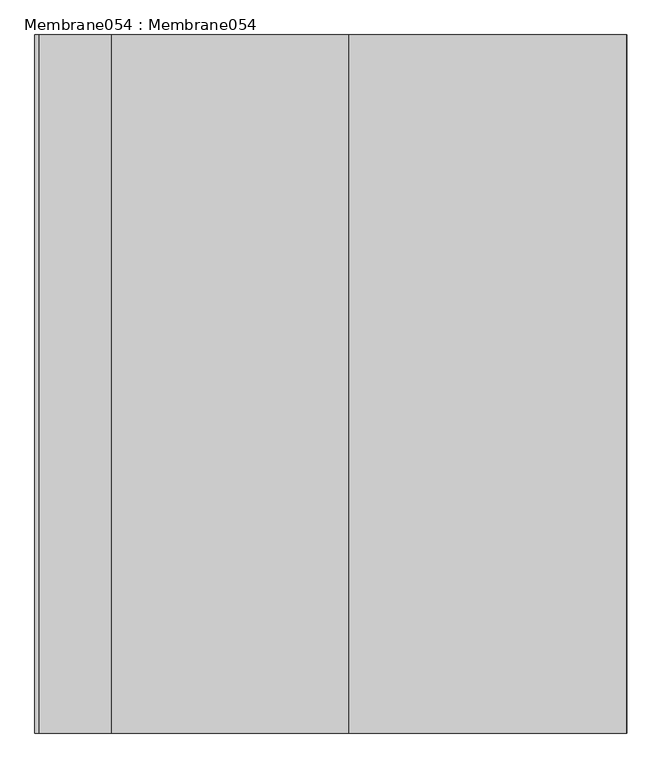
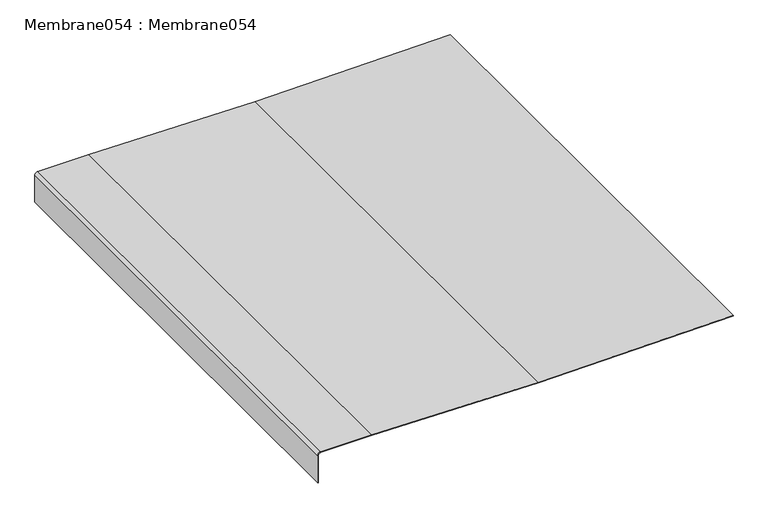
"""IFC4 building model written with IfcOpenShell, lengths in millimetres: proxy geometry, Membrane054 : Membrane054."""

from ifc_helpers import new_model, si_unit, point, frame, frame_2d, origin, place, context, project, spatial, polyline, circle_curve, trimmed, segment, composite_curve, outline, extrude, source, transform, mapped, element, save


def membrane054_membrane054_4ee8488c(model_context):
    return source(origin(), model_context, "Body", "SweptSolid", [
        extrude(outline(composite_curve([segment(trimmed(circle_curve(frame_2d((40233.3001163, -2781.9755019)), 10.0), [point((40233.3001163, -2791.9755019))], [point((40243.3001163, -2781.9755019))], True, "CARTESIAN"), True, "CONTINUOUS"), segment(polyline([(40243.3001163, -2781.9755019), (40243.3001163, -2573.6408736), (40233.5063967, -1893.5405923), (40243.30425, -1097.059185), (40245.3040987, -1097.083786), (40235.5065738, -1893.5384937), (40245.3001163, -2573.6264742), (40245.3001163, -2781.9755019)]), True, "CONTINUOUS"), segment(trimmed(circle_curve(frame_2d((40233.3001163, -2781.9755019)), 12.0), [point((40245.3001163, -2781.9755019))], [point((40233.3001163, -2793.9755019))], False, "CARTESIAN"), True, "CONTINUOUS"), segment(polyline([(40233.3001163, -2793.9755019), (40116.5801181, -2793.9755019), (40116.5801181, -2791.9755019), (40233.3001163, -2791.9755019)]), True, "CONTINUOUS")], self_intersect=False)), frame((0.0, -1052.8906574, 0.0), z_axis=(0.0, 1.0, 0.0), x_axis=(0.0, 0.0, 1.0)), (0.0, 0.0, 1.0), 2000.0),
    ])


if __name__ == "__main__":
    model = new_model("IFC4")
    model_context = context("Model", 3, world=origin())
    ifc_project = project(units=[si_unit("LENGTHUNIT", "METRE", prefix="MILLI")], contexts=[model_context])
    site = spatial("IfcSite", under=ifc_project)
    building = spatial("IfcBuilding", under=site)
    placement = place(None, origin())
    membrane054_membrane054_shape = membrane054_membrane054_4ee8488c(model_context)
    element("IfcBuildingElementProxy", 1, Name="Membrane054 : Membrane054", ObjectType="Membrane054 : Membrane054", at=placement, inside=building, context=model_context, shape_type="MappedRepresentation", body=[
        mapped(membrane054_membrane054_shape, transform((0.0, 0.0, 0.0), x_axis=(1.0, 0.0, 0.0), y_axis=(0.0, 1.0, 0.0), z_axis=(0.0, 0.0, 1.0))),
    ])
    save(model, "model.ifc")

# Revit data of these elements
# Type "Membrane054 : Membrane054"
#   NameOverride = "Membrane054"
# Element 1 (IfcBuildingElementProxy, "Membrane054 : Membrane054")
#   Materials on its faces: "THREE PLY BUILT UP ROOF MEMBRANE"
# Materials
#   "THREE PLY BUILT UP ROOF MEMBRANE": class "Unassigned", colour RGB 63 63 63, transparency 0
